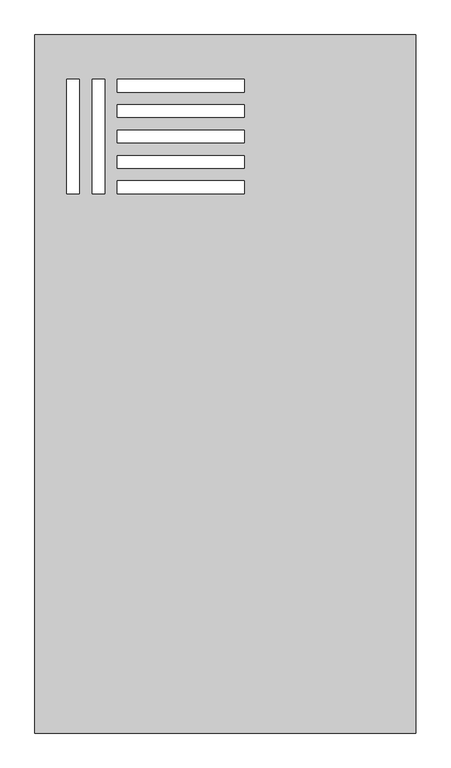
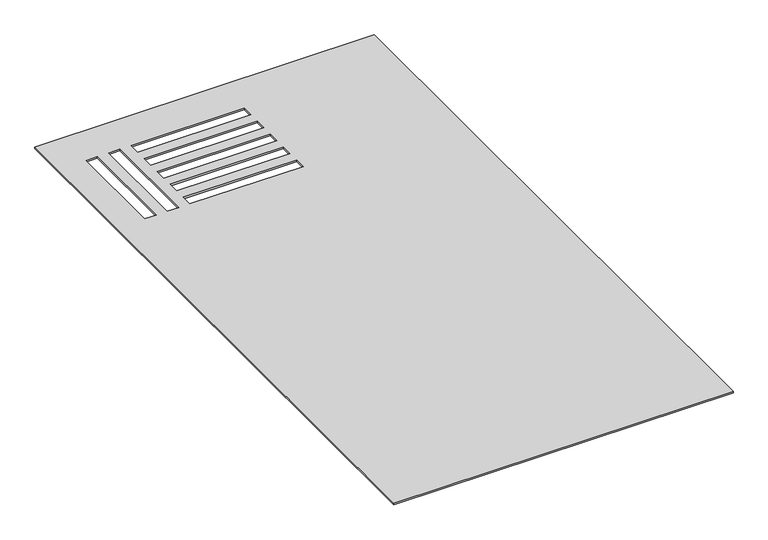
"""IFC4 building model written with IfcOpenShell, lengths in millimetres: proxy geometry, TSP Geyser Electrcical 250L : TSP Geyser Electrcical 250L."""

from ifc_helpers import new_model, si_unit, origin, origin_with_axes, place, context, project, spatial, polyline, outline, extrude, source, transform, mapped, element, save


def electrical_fixtures_8490393c(model_context):
    return source(origin(), model_context, "Body", "SweptSolid", [
        extrude(outline(polyline([(-600.0, 600.0), (0.0, 600.0), (0.0, -500.0), (-600.0, -500.0), (-600.0, 600.0)]), holes=[polyline([(-530.0, 530.0), (-550.0, 530.0), (-550.0, 350.0), (-530.0, 350.0), (-530.0, 530.0)]), polyline([(-470.0, 350.0), (-270.0, 350.0), (-270.0, 370.0), (-470.0, 370.0), (-470.0, 350.0)]), polyline([(-470.0, 390.0), (-270.0, 390.0), (-270.0, 410.0), (-470.0, 410.0), (-470.0, 390.0)]), polyline([(-470.0, 430.0), (-270.0, 430.0), (-270.0, 450.0), (-470.0, 450.0), (-470.0, 430.0)]), polyline([(-470.0, 470.0), (-270.0, 470.0), (-270.0, 490.0), (-470.0, 490.0), (-470.0, 470.0)]), polyline([(-470.0, 510.0), (-270.0, 510.0), (-270.0, 530.0), (-470.0, 530.0), (-470.0, 510.0)]), polyline([(-490.0, 530.0), (-510.0, 530.0), (-510.0, 350.0), (-490.0, 350.0), (-490.0, 530.0)])]), origin_with_axes(), (0.0, 0.0, 1.0), 3.0),
    ])


if __name__ == "__main__":
    model = new_model("IFC4")
    model_context = context("Model", 3, world=origin())
    ifc_project = project(units=[si_unit("LENGTHUNIT", "METRE", prefix="MILLI")], contexts=[model_context])
    site = spatial("IfcSite", under=ifc_project)
    building = spatial("IfcBuilding", under=site)
    placement = place(None, origin())
    electrical_fixtures_shape = electrical_fixtures_8490393c(model_context)
    element("IfcBuildingElementProxy", 1, Name="TSP Geyser Electrcical 250L : TSP Geyser Electrcical 250L", ObjectType="TSP Geyser Electrcical 250L : TSP Geyser Electrcical 250L", at=placement, inside=building, context=model_context, shape_type="MappedRepresentation", body=[
        mapped(electrical_fixtures_shape, transform((0.0, 0.0, 0.0), x_axis=(1.0, 0.0, 0.0), y_axis=(0.0, 1.0, 0.0), z_axis=(0.0, 0.0, 1.0))),
    ])
    save(model, "model.ifc")

# Revit data of these elements
# Type "TSP Geyser Electrcical 250L : TSP Geyser Electrcical 250L"
#   Model = "TSP_EGEY250"
#   Default Elevation = 0
# Element 1 (IfcBuildingElementProxy, "TSP Geyser Electrcical 250L : TSP Geyser Electrcical 250L")
#   Materials on its faces: "Aluminum, Anodized Red"
# Materials
#   "Aluminum, Anodized Red": class "Metal", colour RGB 120 120 120, transparency 0, Description = "Anodized aluminum, red", Cost = 0
